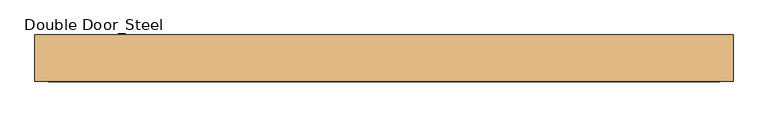
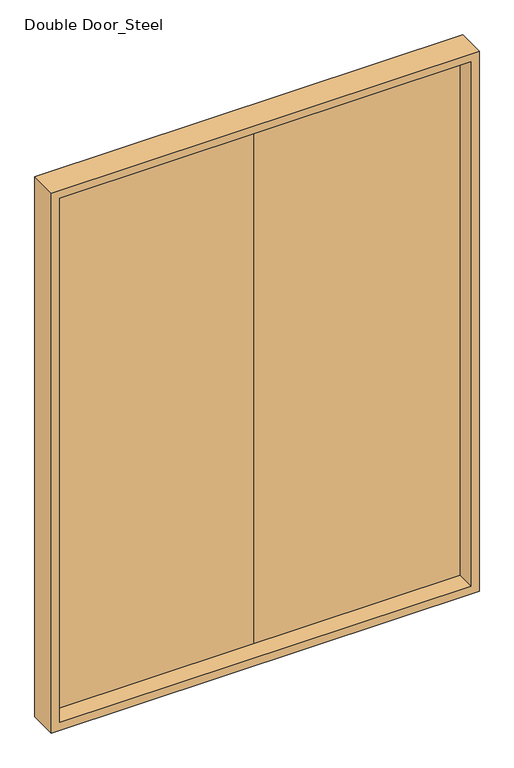
"""IFC4 building model written with IfcOpenShell, lengths in millimetres: door geometry, Double Door_Steel : H_DR_AMB_Double Door_Steel_W2000xH2400."""

from ifc_helpers import new_model, si_unit, frame, origin, place, context, project, spatial, polyline, outline, extrude, faceted_brep, source, transform, mapped, element, save


def double_door_steel_188e4856(model_context):
    return source(origin(), model_context, "Body", "SolidModel", [
        extrude(outline(polyline([(880.0, 20.0), (0.0, 20.0), (0.0, 60.0), (880.0, 60.0), (880.0, 20.0)])), frame((0.0, 0.0, 20.0), z_axis=(0.0, 0.0, 1.0), x_axis=(1.0, 0.0, 0.0)), (0.0, 0.0, 1.0), 2360.0),
        extrude(outline(polyline([(0.0, 20.0), (-880.0, 20.0), (-880.0, 60.0), (0.0, 60.0), (0.0, 20.0)])), frame((0.0, 0.0, 20.0), z_axis=(0.0, 0.0, 1.0), x_axis=(1.0, 0.0, 0.0)), (0.0, 0.0, 1.0), 2360.0),
        faceted_brep([(900.0, -60.0, 2400.0), (900.0, 60.0, 2400.0), (-900.0, 60.0, 2400.0), (-900.0, -60.0, 2400.0), (865.0, 20.0, 2365.0), (865.0, -60.0, 2365.0), (-865.0, -60.0, 2365.0), (-865.0, 20.0, 2365.0), (880.0, 60.0, 2380.0), (880.0, 20.0, 2380.0), (-880.0, 20.0, 2380.0), (-880.0, 60.0, 2380.0), (-900.0, 60.0, 0.0), (-900.0, -60.0, 0.0), (-865.0, -60.0, 35.0), (-865.0, 20.0, 35.0), (-880.0, 20.0, 20.0), (-880.0, 60.0, 20.0), (900.0, 60.0, 0.0), (880.0, 60.0, 20.0), (900.0, -60.0, 0.0), (865.0, -60.0, 35.0), (865.0, 20.0, 35.0), (880.0, 20.0, 20.0)], [[[0, 1, 2, 3]], [[4, 5, 6, 7]], [[8, 9, 10, 11]], [[3, 2, 12, 13]], [[7, 6, 14, 15]], [[11, 10, 16, 17]], [[18, 12, 2, 1], [8, 11, 17, 19]], [[13, 12, 18, 20]], [[0, 3, 13, 20], [21, 14, 6, 5]], [[15, 14, 21, 22]], [[23, 16, 10, 9], [4, 7, 15, 22]], [[17, 16, 23, 19]], [[20, 18, 1, 0]], [[22, 21, 5, 4]], [[19, 23, 9, 8]]]),
    ])


if __name__ == "__main__":
    model = new_model("IFC4")
    model_context = context("Model", 3, world=origin())
    ifc_project = project(units=[si_unit("LENGTHUNIT", "METRE", prefix="MILLI")], contexts=[model_context])
    site = spatial("IfcSite", under=ifc_project)
    building = spatial("IfcBuilding", under=site)
    placement = place(None, origin())
    double_door_steel_shape = double_door_steel_188e4856(model_context)
    element("IfcDoor", 1, ObjectType="Double Door_Steel : H_DR_AMB_Double Door_Steel_W2000xH2400", at=placement, inside=building, context=model_context, shape_type="MappedRepresentation", body=[
        mapped(double_door_steel_shape, transform((0.0, 0.0, 0.0), x_axis=(1.0, 0.0, 0.0), y_axis=(0.0, 1.0, 0.0), z_axis=(0.0, 0.0, 1.0))),
    ])
    save(model, "model.ifc")

# Revit data of these elements
# Type "Double Door_Steel : H_DR_AMB_Double Door_Steel_W2000xH2400"
#   Type Mark = "362"
#   프레임 = ""
#   철물 = ""
#   유리/마감 = ""
#   위치/개소 = ""
#   부호 = "1/SD"
#   문번호 = ""
#   문기호 = "SD"
#   Analytic Construction = "<None>"
#   Height = 2400 mm
#   Width = 1800 mm
#   Define Thermal Properties by = 1
#   문 틀 = none
#   문 = none
#   Function = (empty or 0)
#   Assembly Code = ""
#   Wall Closure = (empty or 0)
